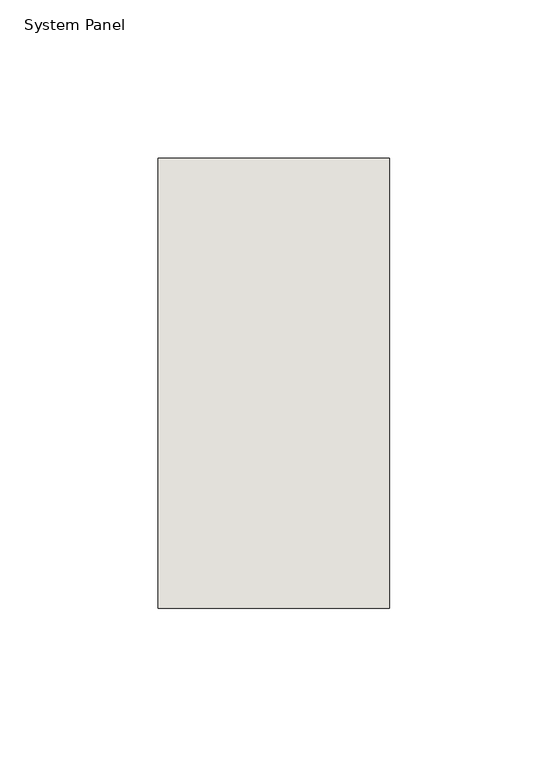
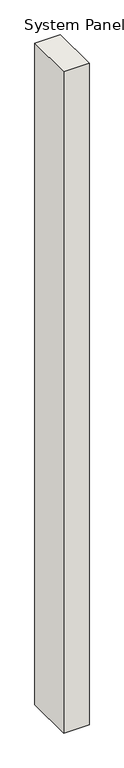
"""IFC4 building model written with IfcOpenShell, lengths in millimetres: wall geometry, System Panel : NLRS_21_CWP_hsb-vulling minerale wol 142 _gen_rsf."""

from ifc_helpers import new_model, si_unit, origin, origin_with_axes, place, context, project, spatial, polyline, outline, extrude, source, transform, mapped, element, save


def system_panel_19d5cf6b(model_context):
    return source(origin(), model_context, "Body", "SweptSolid", [
        extrude(outline(polyline([(36.5, -71.0), (-36.5, -71.0), (-36.5, 71.0), (36.5, 71.0), (36.5, -71.0)])), origin_with_axes(), (0.0, 0.0, 1.0), 2000.0),
    ])


if __name__ == "__main__":
    model = new_model("IFC4")
    model_context = context("Model", 3, world=origin())
    ifc_project = project(units=[si_unit("LENGTHUNIT", "METRE", prefix="MILLI")], contexts=[model_context])
    site = spatial("IfcSite", under=ifc_project)
    building = spatial("IfcBuilding", under=site)
    placement = place(None, origin())
    system_panel_shape = system_panel_19d5cf6b(model_context)
    element("IfcWall", 1, ObjectType="System Panel : NLRS_21_CWP_hsb-vulling minerale wol 142 _gen_rsf", at=placement, inside=building, context=model_context, shape_type="MappedRepresentation", body=[
        mapped(system_panel_shape, transform((0.0, 0.0, 0.0), x_axis=(1.0, 0.0, 0.0), y_axis=(0.0, 1.0, 0.0), z_axis=(0.0, 0.0, 1.0))),
    ])
    save(model, "model.ifc")

# Revit data of these elements
# Type "System Panel : NLRS_21_CWP_hsb-vulling minerale wol 142 _gen_rsf"
#   Type IfcGUID = "07M7mRoiH1CR8m_RSKIwpC"
#   Assembly Code = "21.23"
#   IfcExportAs = "IfcWall"
# Element 1 (IfcWall, "System Panel : NLRS_21_CWP_hsb-vulling minerale wol 142 _gen_rsf")
#   Materials on its faces: "NLRS_m1_isolatie minerale wol_gen_rsf"
# Materials
#   "NLRS_m1_isolatie minerale wol_gen_rsf": class "M - Anorganische materialen", colour RGB 200 200 140, transparency 0, Keynote = "m1", Manufacturer = "Revit Standards Foundation", URL = "www.revitstandards.org", Description = "isolatie minerale wol", Cost = 0
